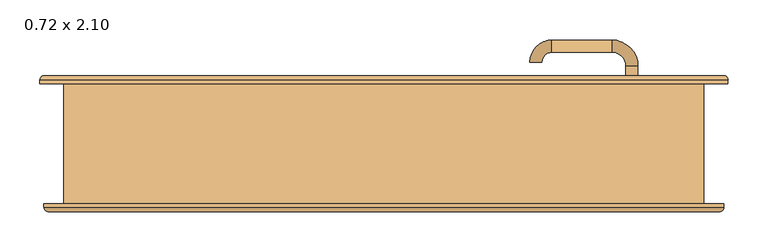
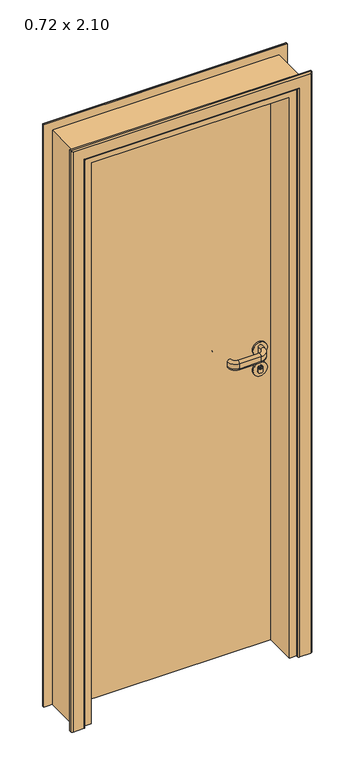
"""IFC4 building model written with IfcOpenShell, lengths in millimetres: door geometry, CC_PORTA ABRIR_1 FOLHA LISA : 0.72 x 2.10."""

from ifc_helpers import new_model, si_unit, point, frame, frame_2d, origin, origin_with_axes, place, context, project, spatial, polyline, circle_curve, ellipse_curve, trimmed, segment, composite_curve, outline, extrude, faceted_brep, source, transform, mapped, element, save
from ifc_brep_helpers import plane_surface, cylinder_surface, revolved_surface, advanced_brep


def door_0_72_x_2_10_9be13891(model_context):
    return source(origin(), model_context, "Body", "SolidModel", [
        advanced_brep(
        [(302.5, 40.0, 1091.5062746), (302.5, 40.0, 1108.3826844), (317.5, 40.0, 1108.3826844), (317.5, 40.0, 1091.5062746), (317.5, 18.0, 1108.3826844), (317.5, 18.0, 1091.5062746), (302.5, 18.0, 1091.5062746), (302.5, 18.0, 1108.3826844), (285.0, -14.5, 1108.3826844), (210.0, -14.5, 1108.3826844), (210.0, -14.5, 1091.5062746), (285.0, -14.5, 1091.5062746), (285.0, 0.5, 1091.5062746), (210.0, 0.5, 1091.5062746), (210.0, 0.5, 1108.3826844), (285.0, 0.5, 1108.3826844), (197.5, 13.0, 1091.5062746), (182.5, 13.0, 1091.5062746), (182.5, 13.0, 1108.3826844), (197.5, 13.0, 1108.3826844)],
        [
            (0, 1),
            (1, 2, circle_curve(frame((310.0, 40.0, 1108.3826844), z_axis=(0.0, 1.0, 0.0), x_axis=(0.0, 0.0, 1.0)), 7.5)),
            (2, 3),
            (3, 0, circle_curve(frame((310.0, 40.0, 1091.5062746), z_axis=(0.0, 1.0, 0.0), x_axis=(0.0, 0.0, 1.0)), 7.5)),
            (2, 4),
            (4, 5),
            (5, 3),
            (0, 6),
            (6, 7),
            (7, 1),
            (8, 9),
            (9, 10),
            (10, 11),
            (11, 8),
            (12, 13),
            (13, 14),
            (14, 15),
            (15, 12),
            (5, 6, circle_curve(frame((310.0, 18.0, 1091.5062746), z_axis=(0.0, 1.0, 0.0), x_axis=(0.0, 0.0, 1.0)), 7.5)),
            (7, 4, circle_curve(frame((310.0, 18.0, 1108.3826844), z_axis=(0.0, 1.0, 0.0), x_axis=(0.0, 0.0, 1.0)), 7.5)),
            (10, 13, circle_curve(frame((210.0, -7.0, 1091.5062746), z_axis=(1.0, 0.0, 0.0), x_axis=(0.0, 0.0, 1.0)), 7.5)),
            (12, 11, circle_curve(frame((285.0, -7.0, 1091.5062746), z_axis=(-1.0, 0.0, 0.0), x_axis=(0.0, 0.0, 1.0)), 7.5)),
            (14, 9, circle_curve(frame((210.0, -7.0, 1108.3826844), z_axis=(1.0, 0.0, 0.0), x_axis=(0.0, 0.0, 1.0)), 7.5)),
            (8, 15, circle_curve(frame((285.0, -7.0, 1108.3826844), z_axis=(-1.0, 0.0, 0.0), x_axis=(0.0, 0.0, 1.0)), 7.5)),
            (12, 6, circle_curve(frame((285.0, 18.0, 1091.5062746), z_axis=(0.0, 0.0, 1.0), x_axis=(1.0, 0.0, 0.0)), 17.5)),
            (5, 11, circle_curve(frame((285.0, 18.0, 1091.5062746), z_axis=(0.0, 0.0, -1.0), x_axis=(1.0, 0.0, 0.0)), 32.5)),
            (4, 8, circle_curve(frame((285.0, 18.0, 1108.3826844), z_axis=(0.0, 0.0, -1.0), x_axis=(1.0, 0.0, 0.0)), 32.5)),
            (7, 15, circle_curve(frame((285.0, 18.0, 1108.3826844), z_axis=(0.0, 0.0, -1.0), x_axis=(1.0, 0.0, 0.0)), 17.5)),
            (16, 17, circle_curve(frame((190.0, 13.0, 1091.5062746), z_axis=(0.0, 1.0, 0.0), x_axis=(0.0, 0.0, 1.0)), 7.5)),
            (17, 18),
            (18, 19, circle_curve(frame((190.0, 13.0, 1108.3826844), z_axis=(0.0, 1.0, 0.0), x_axis=(0.0, 0.0, 1.0)), 7.5)),
            (19, 16),
            (16, 13, circle_curve(frame((210.0, 13.0, 1091.5062746), z_axis=(0.0, 0.0, 1.0), x_axis=(0.0, -1.0, 0.0)), 12.5)),
            (10, 17, circle_curve(frame((210.0, 13.0, 1091.5062746), z_axis=(0.0, 0.0, -1.0), x_axis=(0.0, -1.0, 0.0)), 27.5)),
            (9, 18, circle_curve(frame((210.0, 13.0, 1108.3826844), z_axis=(0.0, 0.0, -1.0), x_axis=(0.0, -1.0, 0.0)), 27.5)),
            (14, 19, circle_curve(frame((210.0, 13.0, 1108.3826844), z_axis=(0.0, 0.0, -1.0), x_axis=(0.0, -1.0, 0.0)), 12.5)),
        ],
        [
            plane_surface(frame((310.0, 40.0, 1099.9444795), z_axis=(0.0, 1.0, 0.0), x_axis=(0.0, 0.0, 1.0))),
            plane_surface(frame((317.5, 40.0, 1091.5062746), z_axis=(1.0, 0.0, 0.0), x_axis=(0.0, -1.0, 0.0))),
            plane_surface(frame((302.5, 40.0, 1108.3826844), z_axis=(-1.0, 0.0, 0.0), x_axis=(0.0, -1.0, 0.0))),
            plane_surface(frame((285.0, -14.5, 1091.5062746), z_axis=(0.0, -1.0, 0.0), x_axis=(-1.0, 0.0, 0.0))),
            plane_surface(frame((285.0, 0.5, 1108.3826844), z_axis=(0.0, 1.0, 0.0), x_axis=(-1.0, 0.0, 0.0))),
            cylinder_surface(frame((310.0, 40.0, 1091.5062746), z_axis=(0.0, 1.0, 0.0), x_axis=(0.0, 0.0, 1.0)), 7.5),
            cylinder_surface(frame((310.0, 40.0, 1108.3826844), z_axis=(0.0, 1.0, 0.0), x_axis=(0.0, 0.0, 1.0)), 7.5),
            cylinder_surface(frame((285.0, -7.0, 1091.5062746), z_axis=(1.0, 0.0, 0.0), x_axis=(0.0, 0.0, 1.0)), 7.5),
            cylinder_surface(frame((285.0, -7.0, 1108.3826844), z_axis=(1.0, 0.0, 0.0), x_axis=(0.0, 0.0, 1.0)), 7.5),
            revolved_surface(trimmed(ellipse_curve(frame((310.0, 18.0, 1091.5062746), z_axis=(0.0, -1.0, 0.0), x_axis=(0.0, 0.0, 1.0)), 7.5, 7.5), [point((302.5, 18.0, 1091.5062746))], [point((317.5, 18.0, 1091.5062746))], True, "CARTESIAN"), (285.0, 18.0, 1099.9444795), (0.0, 0.0, 1.0)),
            cylinder_surface(frame((285.0, 18.0, 1099.9444795), z_axis=(0.0, 0.0, 1.0), x_axis=(1.0, 0.0, 0.0)), 32.5),
            revolved_surface(trimmed(ellipse_curve(frame((310.0, 18.0, 1108.3826844), z_axis=(0.0, -1.0, 0.0), x_axis=(0.0, 0.0, 1.0)), 7.5, 7.5), [point((317.5, 18.0, 1108.3826844))], [point((302.5, 18.0, 1108.3826844))], True, "CARTESIAN"), (285.0, 18.0, 1099.9444795), (0.0, 0.0, 1.0)),
            revolved_surface(polyline([(302.5, 18.0, 1108.3826844), (302.5, 18.0, 1091.5062746)]), (285.0, 18.0, 1099.9444795), (0.0, 0.0, 1.0)),
            plane_surface(frame((190.0, 13.0, 1099.9444795), z_axis=(0.0, 1.0, 0.0), x_axis=(0.0, 0.0, 1.0))),
            revolved_surface(trimmed(ellipse_curve(frame((210.0, -7.0, 1091.5062746), z_axis=(-1.0, 0.0, 0.0), x_axis=(0.0, 0.0, 1.0)), 7.5, 7.5), [point((210.0, 0.5, 1091.5062746))], [point((210.0, -14.5, 1091.5062746))], True, "CARTESIAN"), (210.0, 13.0, 1099.9444795), (0.0, 0.0, 1.0)),
            cylinder_surface(frame((210.0, 13.0, 1099.9444795), z_axis=(0.0, 0.0, 1.0), x_axis=(0.0, -1.0, 0.0)), 27.5),
            revolved_surface(trimmed(ellipse_curve(frame((210.0, -7.0, 1108.3826844), z_axis=(-1.0, 0.0, 0.0), x_axis=(0.0, 0.0, 1.0)), 7.5, 7.5), [point((210.0, -14.5, 1108.3826844))], [point((210.0, 0.5, 1108.3826844))], True, "CARTESIAN"), (210.0, 13.0, 1099.9444795), (0.0, 0.0, 1.0)),
            revolved_surface(polyline([(210.0, 0.5, 1108.3826844), (210.0, 0.5, 1091.5062746)]), (210.0, 13.0, 1099.9444795), (0.0, 0.0, 1.0)),
        ],
        [
            (0, [[1, 2, 3, 4]]),
            (1, [[5, 6, 7, -3]]),
            (2, [[8, 9, 10, -1]]),
            (3, [[11, 12, 13, 14]]),
            (4, [[15, 16, 17, 18]]),
            (5, [[-7, 19, -8, -4]]),
            (6, [[-10, 20, -5, -2]]),
            (7, [[-13, 21, -15, 22]]),
            (8, [[-17, 23, -11, 24]]),
            (9, [[-22, 25, -19, 26]]),
            (10, [[-14, -26, -6, 27]]),
            (11, [[-24, -27, -20, 28]]),
            (12, [[-18, -28, -9, -25]]),
            (13, [[29, 30, 31, 32]]),
            (14, [[-29, 33, -21, 34]]),
            (15, [[-30, -34, -12, 35]]),
            (16, [[-31, -35, -23, 36]]),
            (17, [[-32, -36, -16, -33]]),
        ],
    ),
        extrude(outline(polyline([(311.0, 40.0), (311.0, 30.9), (309.0, 30.9), (309.0, 40.0), (311.0, 40.0)])), frame((0.0, 0.0, 1027.9555433), z_axis=(0.0, 0.0, 1.0), x_axis=(1.0, 0.0, 0.0)), (0.0, 0.0, 1.0), 7.8071257),
        extrude(outline(composite_curve([segment(trimmed(circle_curve(frame_2d((1031.5611613, 310.0)), 5.0), [point((1036.5611613, 310.0))], [point((1026.5611613, 310.0))], False, "CARTESIAN"), True, "CONTINUOUS"), segment(trimmed(circle_curve(frame_2d((1031.5611613, 310.0)), 5.0), [point((1026.5611613, 310.0))], [point((1036.5611613, 310.0))], False, "CARTESIAN"), True, "CONTINUOUS")], self_intersect=False), holes=[polyline([(1035.7626689, 311.0), (1027.9555433, 311.0), (1027.9555433, 309.0), (1035.7626689, 309.0), (1035.7626689, 311.0)])]), frame((0.0, 30.0, 0.0), z_axis=(0.0, 1.0, 0.0), x_axis=(0.0, 0.0, 1.0)), (0.0, 0.0, 1.0), 10.0),
        extrude(outline(composite_curve([segment(polyline([(1033.4817325, 302.5), (1016.4817325, 302.5)]), True, "CONTINUOUS"), segment(trimmed(circle_curve(frame_2d((1016.4817325, 306.5)), 4.0), [point((1016.4817325, 302.5))], [point((1012.4817325, 306.5))], False, "CARTESIAN"), True, "CONTINUOUS"), segment(polyline([(1012.4817325, 306.5), (1012.4817325, 313.5)]), True, "CONTINUOUS"), segment(trimmed(circle_curve(frame_2d((1016.4817325, 313.5)), 4.0), [point((1012.4817325, 313.5))], [point((1016.4817325, 317.5))], False, "CARTESIAN"), True, "CONTINUOUS"), segment(polyline([(1016.4817325, 317.5), (1033.4817325, 317.5)]), True, "CONTINUOUS"), segment(trimmed(circle_curve(frame_2d((1033.4817325, 313.5)), 4.0), [point((1033.4817325, 317.5))], [point((1037.4817325, 313.5))], False, "CARTESIAN"), True, "CONTINUOUS"), segment(polyline([(1037.4817325, 313.5), (1037.4817325, 306.5)]), True, "CONTINUOUS"), segment(trimmed(circle_curve(frame_2d((1033.4817325, 306.5)), 4.0), [point((1037.4817325, 306.5))], [point((1033.4817325, 302.5))], False, "CARTESIAN"), True, "CONTINUOUS")], self_intersect=False)), frame((0.0, 31.0, 0.0), z_axis=(0.0, 1.0, 0.0), x_axis=(0.0, 0.0, 1.0)), (0.0, 0.0, 1.0), 9.0),
        extrude(outline(composite_curve([segment(trimmed(circle_curve(frame_2d((1099.9444795, 310.0)), 25.0), [point((1124.9444795, 310.0))], [point((1074.9444795, 310.0))], False, "CARTESIAN"), True, "CONTINUOUS"), segment(trimmed(circle_curve(frame_2d((1099.9444795, 310.0)), 25.0), [point((1074.9444795, 310.0))], [point((1124.9444795, 310.0))], False, "CARTESIAN"), True, "CONTINUOUS")], self_intersect=False)), frame((0.0, 34.0, 0.0), z_axis=(0.0, 1.0, 0.0), x_axis=(0.0, 0.0, 1.0)), (0.0, 0.0, 1.0), 6.0),
        extrude(outline(composite_curve([segment(trimmed(circle_curve(frame_2d((1024.9444795, 310.0)), 25.0), [point((1049.9444795, 310.0))], [point((999.9444795, 310.0))], False, "CARTESIAN"), True, "CONTINUOUS"), segment(trimmed(circle_curve(frame_2d((1024.9444795, 310.0)), 25.0), [point((999.9444795, 310.0))], [point((1049.9444795, 310.0))], False, "CARTESIAN"), True, "CONTINUOUS")], self_intersect=False), holes=[composite_curve([segment(trimmed(circle_curve(frame_2d((1033.4817325, 313.5)), 4.0), [point((1037.4817325, 313.5))], [point((1033.4817325, 317.5))], True, "CARTESIAN"), True, "CONTINUOUS"), segment(polyline([(1033.4817325, 317.5), (1016.4817325, 317.5)]), True, "CONTINUOUS"), segment(trimmed(circle_curve(frame_2d((1016.4817325, 313.5)), 4.0), [point((1016.4817325, 317.5))], [point((1012.4817325, 313.5))], True, "CARTESIAN"), True, "CONTINUOUS"), segment(polyline([(1012.4817325, 313.5), (1012.4817325, 306.5)]), True, "CONTINUOUS"), segment(trimmed(circle_curve(frame_2d((1016.4817325, 306.5)), 4.0), [point((1012.4817325, 306.5))], [point((1016.4817325, 302.5))], True, "CARTESIAN"), True, "CONTINUOUS"), segment(polyline([(1016.4817325, 302.5), (1033.4817325, 302.5)]), True, "CONTINUOUS"), segment(trimmed(circle_curve(frame_2d((1033.4817325, 306.5)), 4.0), [point((1033.4817325, 302.5))], [point((1037.4817325, 306.5))], True, "CARTESIAN"), True, "CONTINUOUS"), segment(polyline([(1037.4817325, 306.5), (1037.4817325, 313.5)]), True, "CONTINUOUS")], self_intersect=False)]), frame((0.0, 34.0, 0.0), z_axis=(0.0, 1.0, 0.0), x_axis=(0.0, 0.0, 1.0)), (0.0, 0.0, 1.0), 6.0),
        extrude(outline(polyline([(311.0, 84.1), (311.0, 75.0), (309.0, 75.0), (309.0, 84.1), (311.0, 84.1)])), frame((0.0, 0.0, 1027.9555433), z_axis=(0.0, 0.0, 1.0), x_axis=(1.0, 0.0, 0.0)), (0.0, 0.0, 1.0), 7.8071257),
        advanced_brep(
        [(310.0, 85.0, 1036.5611613), (310.0, 85.0, 1026.5611613), (311.0, 85.0, 1035.7626689), (309.0, 85.0, 1035.7626689), (309.0, 85.0, 1027.9555433), (311.0, 85.0, 1027.9555433), (310.0, 75.0, 1049.9444795), (310.0, 75.0, 999.9444795), (310.0, 84.0, 1026.5611613), (310.0, 84.0, 1036.5611613), (311.0, 84.0, 1027.9555433), (311.0, 84.0, 1035.7626689), (309.0, 84.0, 1027.9555433), (309.0, 84.0, 1035.7626689), (302.5, 84.0, 1033.4817325), (306.5, 84.0, 1037.4817325), (313.5, 84.0, 1037.4817325), (317.5, 84.0, 1033.4817325), (317.5, 84.0, 1016.4817325), (313.5, 84.0, 1012.4817325), (306.5, 84.0, 1012.4817325), (302.5, 84.0, 1016.4817325), (302.5, 81.0, 1016.4817325), (302.5, 81.0, 1033.4817325), (306.5, 81.0, 1012.4817325), (313.5, 81.0, 1012.4817325), (317.5, 81.0, 1016.4817325), (317.5, 81.0, 1033.4817325), (313.5, 81.0, 1037.4817325), (306.5, 81.0, 1037.4817325), (310.0, 81.0, 1049.9444795), (310.0, 81.0, 999.9444795)],
        [
            (0, 1, circle_curve(frame((310.0, 85.0, 1031.5611613), z_axis=(0.0, 1.0, 0.0), x_axis=(0.0, 0.0, -1.0)), 5.0)),
            (1, 0, circle_curve(frame((310.0, 85.0, 1031.5611613), z_axis=(0.0, 1.0, 0.0), x_axis=(0.0, 0.0, -1.0)), 5.0)),
            (2, 3),
            (3, 4),
            (4, 5),
            (5, 2),
            (6, 7, circle_curve(frame((310.0, 75.0, 1024.9444795), z_axis=(0.0, -1.0, 0.0), x_axis=(0.0, 0.0, -1.0)), 25.0)),
            (7, 6, circle_curve(frame((310.0, 75.0, 1024.9444795), z_axis=(0.0, -1.0, 0.0), x_axis=(0.0, 0.0, -1.0)), 25.0)),
            (1, 8),
            (8, 9, circle_curve(frame((310.0, 84.0, 1031.5611613), z_axis=(0.0, 1.0, 0.0), x_axis=(0.0, 0.0, -1.0)), 5.0)),
            (9, 0),
            (9, 8, circle_curve(frame((310.0, 84.0, 1031.5611613), z_axis=(0.0, 1.0, 0.0), x_axis=(0.0, 0.0, -1.0)), 5.0)),
            (5, 10),
            (10, 11),
            (11, 2),
            (4, 12),
            (12, 10),
            (3, 13),
            (13, 12),
            (11, 13),
            (14, 15, circle_curve(frame((306.5, 84.0, 1033.4817325), z_axis=(0.0, 1.0, 0.0), x_axis=(0.0, 0.0, -1.0)), 4.0)),
            (15, 16),
            (16, 17, circle_curve(frame((313.5, 84.0, 1033.4817325), z_axis=(0.0, 1.0, 0.0), x_axis=(0.0, 0.0, -1.0)), 4.0)),
            (17, 18),
            (18, 19, circle_curve(frame((313.5, 84.0, 1016.4817325), z_axis=(0.0, 1.0, 0.0), x_axis=(0.0, 0.0, -1.0)), 4.0)),
            (19, 20),
            (20, 21, circle_curve(frame((306.5, 84.0, 1016.4817325), z_axis=(0.0, 1.0, 0.0), x_axis=(0.0, 0.0, -1.0)), 4.0)),
            (21, 14),
            (21, 22),
            (22, 23),
            (23, 14),
            (20, 24),
            (24, 22, circle_curve(frame((306.5, 81.0, 1016.4817325), z_axis=(0.0, 1.0, 0.0), x_axis=(0.0, 0.0, -1.0)), 4.0)),
            (19, 25),
            (25, 24),
            (18, 26),
            (26, 25, circle_curve(frame((313.5, 81.0, 1016.4817325), z_axis=(0.0, 1.0, 0.0), x_axis=(0.0, 0.0, -1.0)), 4.0)),
            (17, 27),
            (27, 26),
            (16, 28),
            (28, 27, circle_curve(frame((313.5, 81.0, 1033.4817325), z_axis=(0.0, 1.0, 0.0), x_axis=(0.0, 0.0, -1.0)), 4.0)),
            (15, 29),
            (29, 28),
            (23, 29, circle_curve(frame((306.5, 81.0, 1033.4817325), z_axis=(0.0, 1.0, 0.0), x_axis=(0.0, 0.0, -1.0)), 4.0)),
            (30, 31, circle_curve(frame((310.0, 81.0, 1024.9444795), z_axis=(0.0, 1.0, 0.0), x_axis=(0.0, 0.0, -1.0)), 25.0)),
            (31, 30, circle_curve(frame((310.0, 81.0, 1024.9444795), z_axis=(0.0, 1.0, 0.0), x_axis=(0.0, 0.0, -1.0)), 25.0)),
            (31, 7),
            (6, 30),
        ],
        [
            plane_surface(frame((310.0, 85.0, 1026.5611613), z_axis=(0.0, 1.0, 0.0), x_axis=(1.0, 0.0, 0.0))),
            plane_surface(frame((310.0, 75.0, 1026.5611613), z_axis=(0.0, -1.0, 0.0), x_axis=(-1.0, 0.0, 0.0))),
            cylinder_surface(frame((310.0, 75.0, 1031.5611613), z_axis=(0.0, 1.0, 0.0), x_axis=(0.0, 0.0, -1.0)), 5.0),
            plane_surface(frame((311.0, 85.0, 1035.7626689), z_axis=(-1.0, 0.0, 0.0), x_axis=(0.0, -1.0, 0.0))),
            plane_surface(frame((311.0, 85.0, 1027.9555433), z_axis=(0.0, 0.0, 1.0), x_axis=(0.0, -1.0, 0.0))),
            plane_surface(frame((309.0, 85.0, 1027.9555433), z_axis=(1.0, 0.0, 0.0), x_axis=(0.0, -1.0, 0.0))),
            plane_surface(frame((309.0, 85.0, 1035.7626689), z_axis=(0.0, 0.0, -1.0), x_axis=(0.0, -1.0, 0.0))),
            plane_surface(frame((302.5, 84.0, 1016.4817325), z_axis=(0.0, 1.0, 0.0), x_axis=(0.0, 0.0, -1.0))),
            plane_surface(frame((302.5, 84.0, 1033.4817325), z_axis=(-1.0, 0.0, 0.0), x_axis=(0.0, -1.0, 0.0))),
            cylinder_surface(frame((306.5, 75.0, 1016.4817325), z_axis=(0.0, 1.0, 0.0), x_axis=(0.0, 0.0, -1.0)), 4.0),
            plane_surface(frame((306.5, 84.0, 1012.4817325), z_axis=(0.0, 0.0, -1.0), x_axis=(0.0, -1.0, 0.0))),
            cylinder_surface(frame((313.5, 75.0, 1016.4817325), z_axis=(0.0, 1.0, 0.0), x_axis=(0.0, 0.0, -1.0)), 4.0),
            plane_surface(frame((317.5, 84.0, 1016.4817325), z_axis=(1.0, 0.0, 0.0), x_axis=(0.0, -1.0, 0.0))),
            cylinder_surface(frame((313.5, 75.0, 1033.4817325), z_axis=(0.0, 1.0, 0.0), x_axis=(0.0, 0.0, -1.0)), 4.0),
            plane_surface(frame((313.5, 84.0, 1037.4817325), z_axis=(0.0, 0.0, 1.0), x_axis=(0.0, -1.0, 0.0))),
            cylinder_surface(frame((306.5, 75.0, 1033.4817325), z_axis=(0.0, 1.0, 0.0), x_axis=(0.0, 0.0, -1.0)), 4.0),
            plane_surface(frame((310.0, 81.0, 1074.9444795), z_axis=(0.0, 1.0, 0.0), x_axis=(1.0, 0.0, 0.0))),
            cylinder_surface(frame((310.0, 75.0, 1024.9444795), z_axis=(0.0, 1.0, 0.0), x_axis=(0.0, 0.0, -1.0)), 25.0),
        ],
        [
            (0, [[1, 2], [3, 4, 5, 6]]),
            (1, [[7, 8]]),
            (2, [[9, 10, 11, -2]]),
            (2, [[-11, 12, -9, -1]]),
            (3, [[13, 14, 15, -6]]),
            (4, [[16, 17, -13, -5]]),
            (5, [[18, 19, -16, -4]]),
            (6, [[-15, 20, -18, -3]]),
            (7, [[-17, -19, -20, -14]]),
            (7, [[21, 22, 23, 24, 25, 26, 27, 28], [-12, -10]]),
            (8, [[29, 30, 31, -28]]),
            (9, [[32, 33, -29, -27]]),
            (10, [[34, 35, -32, -26]]),
            (11, [[36, 37, -34, -25]]),
            (12, [[38, 39, -36, -24]]),
            (13, [[40, 41, -38, -23]]),
            (14, [[42, 43, -40, -22]]),
            (15, [[-31, 44, -42, -21]]),
            (16, [[45, 46], [-33, -35, -37, -39, -41, -43, -44, -30]]),
            (17, [[47, -7, 48, -46]]),
            (17, [[-48, -8, -47, -45]]),
        ],
    ),
        advanced_brep(
        [(310.0, 75.0, 1124.9444795), (310.0, 75.0, 1074.9444795), (310.0, 81.0, 1124.9444795), (310.0, 81.0, 1074.9444795)],
        [
            (0, 1, circle_curve(frame((310.0, 75.0, 1099.9444795), z_axis=(0.0, -1.0, 0.0), x_axis=(0.0, 0.0, -1.0)), 25.0)),
            (1, 0, circle_curve(frame((310.0, 75.0, 1099.9444795), z_axis=(0.0, -1.0, 0.0), x_axis=(0.0, 0.0, -1.0)), 25.0)),
            (2, 3, circle_curve(frame((310.0, 81.0, 1099.9444795), z_axis=(0.0, 1.0, 0.0), x_axis=(0.0, 0.0, -1.0)), 25.0)),
            (3, 2, circle_curve(frame((310.0, 81.0, 1099.9444795), z_axis=(0.0, 1.0, 0.0), x_axis=(0.0, 0.0, -1.0)), 25.0)),
            (3, 1),
            (0, 2),
        ],
        [
            plane_surface(frame((310.0, 75.0, 1026.5611613), z_axis=(0.0, -1.0, 0.0), x_axis=(-1.0, 0.0, 0.0))),
            plane_surface(frame((310.0, 81.0, 1074.9444795), z_axis=(0.0, 1.0, 0.0), x_axis=(1.0, 0.0, 0.0))),
            cylinder_surface(frame((310.0, 75.0, 1099.9444795), z_axis=(0.0, 1.0, 0.0), x_axis=(0.0, 0.0, -1.0)), 25.0),
        ],
        [
            (0, [[1, 2]]),
            (1, [[3, 4]]),
            (2, [[5, -1, 6, -4]]),
            (2, [[-6, -2, -5, -3]]),
        ],
    ),
        advanced_brep(
        [(302.5, 75.0, 1108.4382049), (302.5, 75.0, 1091.5617951), (317.5, 75.0, 1091.5617951), (317.5, 75.0, 1108.4382049), (317.5, 97.0, 1091.5617951), (317.5, 97.0, 1108.4382049), (302.5, 97.0, 1108.4382049), (302.5, 97.0, 1091.5617951), (285.0, 129.5, 1091.5617951), (210.0, 129.5, 1091.5617951), (210.0, 129.5, 1108.4382049), (285.0, 129.5, 1108.4382049), (285.0, 114.5, 1108.4382049), (210.0, 114.5, 1108.4382049), (210.0, 114.5, 1091.5617951), (285.0, 114.5, 1091.5617951), (197.5, 102.0, 1108.4382049), (182.5, 102.0, 1108.4382049), (182.5, 102.0, 1091.5617951), (197.5, 102.0, 1091.5617951)],
        [
            (0, 1),
            (1, 2, circle_curve(frame((310.0, 75.0, 1091.5617951), z_axis=(0.0, -1.0, 0.0), x_axis=(-1.0, 0.0, 0.0)), 7.5)),
            (2, 3),
            (3, 0, circle_curve(frame((310.0, 75.0, 1108.4382049), z_axis=(0.0, -1.0, 0.0), x_axis=(-1.0, 0.0, 0.0)), 7.5)),
            (2, 4),
            (4, 5),
            (5, 3),
            (0, 6),
            (6, 7),
            (7, 1),
            (8, 9),
            (9, 10),
            (10, 11),
            (11, 8),
            (12, 13),
            (13, 14),
            (14, 15),
            (15, 12),
            (5, 6, circle_curve(frame((310.0, 97.0, 1108.4382049), z_axis=(0.0, -1.0, 0.0), x_axis=(-1.0, 0.0, 0.0)), 7.5)),
            (7, 4, circle_curve(frame((310.0, 97.0, 1091.5617951), z_axis=(0.0, -1.0, 0.0), x_axis=(-1.0, 0.0, 0.0)), 7.5)),
            (10, 13, circle_curve(frame((210.0, 122.0, 1108.4382049), z_axis=(1.0, 0.0, 0.0), x_axis=(0.0, -1.0, 0.0)), 7.5)),
            (12, 11, circle_curve(frame((285.0, 122.0, 1108.4382049), z_axis=(-1.0, 0.0, 0.0), x_axis=(0.0, -1.0, 0.0)), 7.5)),
            (14, 9, circle_curve(frame((210.0, 122.0, 1091.5617951), z_axis=(1.0, 0.0, 0.0), x_axis=(0.0, -1.0, 0.0)), 7.5)),
            (8, 15, circle_curve(frame((285.0, 122.0, 1091.5617951), z_axis=(-1.0, 0.0, 0.0), x_axis=(0.0, -1.0, 0.0)), 7.5)),
            (12, 6, circle_curve(frame((285.0, 97.0, 1108.4382049), z_axis=(0.0, 0.0, -1.0), x_axis=(1.0, 0.0, 0.0)), 17.5)),
            (5, 11, circle_curve(frame((285.0, 97.0, 1108.4382049), z_axis=(0.0, 0.0, 1.0), x_axis=(1.0, 0.0, 0.0)), 32.5)),
            (4, 8, circle_curve(frame((285.0, 97.0, 1091.5617951), z_axis=(0.0, 0.0, 1.0), x_axis=(1.0, 0.0, 0.0)), 32.5)),
            (7, 15, circle_curve(frame((285.0, 97.0, 1091.5617951), z_axis=(0.0, 0.0, 1.0), x_axis=(1.0, 0.0, 0.0)), 17.5)),
            (16, 17, circle_curve(frame((190.0, 102.0, 1108.4382049), z_axis=(0.0, -1.0, 0.0), x_axis=(1.0, 0.0, 0.0)), 7.5)),
            (17, 18),
            (18, 19, circle_curve(frame((190.0, 102.0, 1091.5617951), z_axis=(0.0, -1.0, 0.0), x_axis=(1.0, 0.0, 0.0)), 7.5)),
            (19, 16),
            (16, 13, circle_curve(frame((210.0, 102.0, 1108.4382049), z_axis=(0.0, 0.0, -1.0), x_axis=(0.0, 1.0, 0.0)), 12.5)),
            (10, 17, circle_curve(frame((210.0, 102.0, 1108.4382049), z_axis=(0.0, 0.0, 1.0), x_axis=(0.0, 1.0, 0.0)), 27.5)),
            (9, 18, circle_curve(frame((210.0, 102.0, 1091.5617951), z_axis=(0.0, 0.0, 1.0), x_axis=(0.0, 1.0, 0.0)), 27.5)),
            (14, 19, circle_curve(frame((210.0, 102.0, 1091.5617951), z_axis=(0.0, 0.0, 1.0), x_axis=(0.0, 1.0, 0.0)), 12.5)),
        ],
        [
            plane_surface(frame((310.0, 75.0, 1100.0), z_axis=(0.0, -1.0, 0.0), x_axis=(0.0, 0.0, -1.0))),
            plane_surface(frame((317.5, 75.0, 1108.4382049), z_axis=(1.0, 0.0, 0.0), x_axis=(0.0, 1.0, 0.0))),
            plane_surface(frame((302.5, 75.0, 1091.5617951), z_axis=(-1.0, 0.0, 0.0), x_axis=(0.0, 1.0, 0.0))),
            plane_surface(frame((285.0, 129.5, 1108.4382049), z_axis=(0.0, 1.0, 0.0), x_axis=(-1.0, 0.0, 0.0))),
            plane_surface(frame((285.0, 114.5, 1091.5617951), z_axis=(0.0, -1.0, 0.0), x_axis=(-1.0, 0.0, 0.0))),
            cylinder_surface(frame((310.0, 75.0, 1108.4382049), z_axis=(0.0, -1.0, 0.0), x_axis=(-1.0, 0.0, 0.0)), 7.5),
            cylinder_surface(frame((310.0, 75.0, 1091.5617951), z_axis=(0.0, -1.0, 0.0), x_axis=(-1.0, 0.0, 0.0)), 7.5),
            cylinder_surface(frame((285.0, 122.0, 1108.4382049), z_axis=(1.0, 0.0, 0.0), x_axis=(0.0, -1.0, 0.0)), 7.5),
            cylinder_surface(frame((285.0, 122.0, 1091.5617951), z_axis=(1.0, 0.0, 0.0), x_axis=(0.0, -1.0, 0.0)), 7.5),
            revolved_surface(trimmed(ellipse_curve(frame((310.0, 97.0, 1108.4382049), z_axis=(0.0, 1.0, 0.0), x_axis=(-1.0, 0.0, 0.0)), 7.5, 7.5), [point((302.5, 97.0, 1108.4382049))], [point((317.5, 97.0, 1108.4382049))], True, "CARTESIAN"), (285.0, 97.0, 1100.0), (0.0, 0.0, -1.0)),
            cylinder_surface(frame((285.0, 97.0, 1100.0), z_axis=(0.0, 0.0, -1.0), x_axis=(1.0, 0.0, 0.0)), 32.5),
            revolved_surface(trimmed(ellipse_curve(frame((310.0, 97.0, 1091.5617951), z_axis=(0.0, 1.0, 0.0), x_axis=(-1.0, 0.0, 0.0)), 7.5, 7.5), [point((317.5, 97.0, 1091.5617951))], [point((302.5, 97.0, 1091.5617951))], True, "CARTESIAN"), (285.0, 97.0, 1100.0), (0.0, 0.0, -1.0)),
            revolved_surface(polyline([(302.5, 97.0, 1091.5617951), (302.5, 97.0, 1108.4382049)]), (285.0, 97.0, 1100.0), (0.0, 0.0, -1.0)),
            plane_surface(frame((190.0, 102.0, 1100.0), z_axis=(0.0, -1.0, 0.0), x_axis=(0.0, 0.0, -1.0))),
            revolved_surface(trimmed(ellipse_curve(frame((210.0, 122.0, 1108.4382049), z_axis=(-1.0, 0.0, 0.0), x_axis=(0.0, -1.0, 0.0)), 7.5, 7.5), [point((210.0, 114.5, 1108.4382049))], [point((210.0, 129.5, 1108.4382049))], True, "CARTESIAN"), (210.0, 102.0, 1100.0), (0.0, 0.0, -1.0)),
            cylinder_surface(frame((210.0, 102.0, 1100.0), z_axis=(0.0, 0.0, -1.0), x_axis=(0.0, 1.0, 0.0)), 27.5),
            revolved_surface(trimmed(ellipse_curve(frame((210.0, 122.0, 1091.5617951), z_axis=(-1.0, 0.0, 0.0), x_axis=(0.0, -1.0, 0.0)), 7.5, 7.5), [point((210.0, 129.5, 1091.5617951))], [point((210.0, 114.5, 1091.5617951))], True, "CARTESIAN"), (210.0, 102.0, 1100.0), (0.0, 0.0, -1.0)),
            revolved_surface(polyline([(210.0, 114.5, 1091.5617951), (210.0, 114.5, 1108.4382049)]), (210.0, 102.0, 1100.0), (0.0, 0.0, -1.0)),
        ],
        [
            (0, [[1, 2, 3, 4]]),
            (1, [[5, 6, 7, -3]]),
            (2, [[8, 9, 10, -1]]),
            (3, [[11, 12, 13, 14]]),
            (4, [[15, 16, 17, 18]]),
            (5, [[-7, 19, -8, -4]]),
            (6, [[-10, 20, -5, -2]]),
            (7, [[-13, 21, -15, 22]]),
            (8, [[-17, 23, -11, 24]]),
            (9, [[-22, 25, -19, 26]]),
            (10, [[-14, -26, -6, 27]]),
            (11, [[-24, -27, -20, 28]]),
            (12, [[-18, -28, -9, -25]]),
            (13, [[29, 30, 31, 32]]),
            (14, [[-29, 33, -21, 34]]),
            (15, [[-30, -34, -12, 35]]),
            (16, [[-31, -35, -23, 36]]),
            (17, [[-32, -36, -16, -33]]),
        ],
    ),
        extrude(outline(polyline([(360.0, 75.0), (360.0, 40.0), (-360.0, 40.0), (-360.0, 75.0), (360.0, 75.0)])), origin_with_axes(), (0.0, 0.0, 1.0), 2100.0),
        advanced_brep(
        [(-380.5, -85.0, 0.0), (-419.500573, -85.0, 0.0), (-425.0, -79.500573, 0.0), (-425.0, -75.0, 0.0), (-375.0, -75.0, 0.0), (-375.0, -79.5, 0.0), (-375.0, -79.5, 2115.0), (-380.5, -85.0, 2120.5), (-375.0, -75.0, 2115.0), (-425.0, -75.0, 2165.0), (425.0, -75.0, 2165.0), (425.0, -75.0, 0.0), (375.0, -75.0, 0.0), (375.0, -75.0, 2115.0), (-425.0, -79.500573, 2165.0), (-419.500573, -85.0, 2159.500573), (380.5, -85.0, 2120.5), (380.5, -85.0, 0.0), (419.500573, -85.0, 0.0), (419.500573, -85.0, 2159.500573), (375.0, -79.5, 0.0), (375.0, -79.5, 2115.0), (425.0, -79.500573, 0.0), (425.0, -79.500573, 2165.0)],
        [
            (0, 1),
            (1, 2, circle_curve(frame((-419.500573, -79.500573, 0.0), z_axis=(0.0, 0.0, -1.0), x_axis=(0.0, -1.0, 0.0)), 5.499427)),
            (2, 3),
            (3, 4),
            (4, 5),
            (5, 0, circle_curve(frame((-380.5, -79.5, 0.0), z_axis=(0.0, 0.0, -1.0), x_axis=(0.0, -1.0, 0.0)), 5.5)),
            (5, 6),
            (6, 7, ellipse_curve(frame((-380.5, -79.5, 2120.5), z_axis=(-0.7071067811865475, 0.0, -0.7071067811865476), x_axis=(0.7071067811865476, 0.0, -0.7071067811865474)), 7.7781746, 5.5)),
            (7, 0),
            (4, 8),
            (8, 6),
            (3, 9),
            (9, 10),
            (10, 11),
            (11, 12),
            (12, 13),
            (13, 8),
            (2, 14),
            (14, 9),
            (1, 15),
            (15, 14, ellipse_curve(frame((-419.500573, -79.500573, 2159.500573), z_axis=(-0.7071067811865475, 0.0, -0.7071067811865476), x_axis=(0.7071067811865476, 0.0, -0.7071067811865474)), 7.7773642, 5.499427)),
            (7, 16),
            (16, 17),
            (17, 18),
            (18, 19),
            (19, 15),
            (12, 20),
            (20, 21),
            (21, 13),
            (17, 20, circle_curve(frame((380.5, -79.5, 0.0), z_axis=(0.0, 0.0, -1.0), x_axis=(0.0, -1.0, 0.0)), 5.5)),
            (11, 22),
            (22, 18, circle_curve(frame((419.500573, -79.500573, 0.0), z_axis=(0.0, 0.0, -1.0), x_axis=(0.0, -1.0, 0.0)), 5.499427)),
            (23, 22),
            (10, 23),
            (23, 19, ellipse_curve(frame((419.500573, -79.500573, 2159.500573), z_axis=(0.7071067811865475, 0.0, -0.7071067811865475), x_axis=(0.7071067811865474, 0.0, 0.7071067811865477)), 7.7773642, 5.499427)),
            (16, 21, ellipse_curve(frame((380.5, -79.5, 2120.5), z_axis=(0.7071067811865475, 0.0, -0.7071067811865475), x_axis=(0.7071067811865474, 0.0, 0.7071067811865477)), 7.7781746, 5.5)),
            (6, 21),
            (14, 23),
        ],
        [
            plane_surface(frame((-400.0, -75.0, 0.0), z_axis=(0.0, 0.0, -1.0), x_axis=(-1.0, 0.0, 0.0))),
            cylinder_surface(frame((-380.5, -79.5, 0.0), z_axis=(0.0, 0.0, -1.0), x_axis=(0.0, -1.0, 0.0)), 5.5),
            plane_surface(frame((-375.0, -79.5, 0.0), z_axis=(1.0, 0.0, 0.0), x_axis=(0.0, 0.0, 1.0))),
            plane_surface(frame((-375.0, -75.0, 0.0), z_axis=(0.0, 1.0, 0.0), x_axis=(0.0, 0.0, 1.0))),
            plane_surface(frame((-425.0, -75.0, 0.0), z_axis=(-1.0, 0.0, 0.0), x_axis=(0.0, 0.0, 1.0))),
            cylinder_surface(frame((-419.500573, -79.500573, 0.0), z_axis=(0.0, 0.0, -1.0), x_axis=(0.0, -1.0, 0.0)), 5.499427),
            plane_surface(frame((-419.500573, -85.0, 0.0), z_axis=(0.0, -1.0, 0.0), x_axis=(0.0, 0.0, 1.0))),
            plane_surface(frame((375.0, -79.5, 2115.0), z_axis=(-1.0, 0.0, 0.0), x_axis=(0.0, 0.0, -1.0))),
            plane_surface(frame((400.0, -75.0, 0.0), z_axis=(0.0, 0.0, -1.0), x_axis=(1.0, 0.0, 0.0))),
            plane_surface(frame((425.0, -75.0, 2165.0), z_axis=(1.0, 0.0, 0.0), x_axis=(0.0, 0.0, -1.0))),
            cylinder_surface(frame((419.500573, -79.500573, 2140.0), z_axis=(0.0, 0.0, 1.0), x_axis=(0.0, -1.0, 0.0)), 5.499427),
            cylinder_surface(frame((380.5, -79.5, 2140.0), z_axis=(0.0, 0.0, 1.0), x_axis=(0.0, -1.0, 0.0)), 5.5),
            cylinder_surface(frame((-400.0, -79.5, 2120.5), z_axis=(-1.0, 0.0, 0.0), x_axis=(0.0, -1.0, 0.0)), 5.5),
            plane_surface(frame((-375.0, -79.5, 2115.0), z_axis=(0.0, 0.0, -1.0), x_axis=(1.0, 0.0, 0.0))),
            plane_surface(frame((-425.0, -75.0, 2165.0), z_axis=(0.0, 0.0, 1.0), x_axis=(1.0, 0.0, 0.0))),
            cylinder_surface(frame((-400.0, -79.500573, 2159.500573), z_axis=(-1.0, 0.0, 0.0), x_axis=(0.0, -1.0, 0.0)), 5.499427),
        ],
        [
            (0, [[1, 2, 3, 4, 5, 6]]),
            (1, [[7, 8, 9, -6]]),
            (2, [[10, 11, -7, -5]]),
            (3, [[12, 13, 14, 15, 16, 17, -10, -4]]),
            (4, [[18, 19, -12, -3]]),
            (5, [[20, 21, -18, -2]]),
            (6, [[-9, 22, 23, 24, 25, 26, -20, -1]]),
            (7, [[-16, 27, 28, 29]]),
            (8, [[30, -27, -15, 31, 32, -24]]),
            (9, [[33, -31, -14, 34]]),
            (10, [[-25, -32, -33, 35]]),
            (11, [[-28, -30, -23, 36]]),
            (12, [[37, -36, -22, -8]]),
            (13, [[-17, -29, -37, -11]]),
            (14, [[38, -34, -13, -19]]),
            (15, [[-26, -35, -38, -21]]),
        ],
    ),
        advanced_brep(
        [(-380.0, 75.0, 0.0), (-430.0, 75.0, 0.0), (-430.0, 79.5, 0.0), (-424.5, 85.0, 0.0), (-385.5, 85.0, 0.0), (-380.0, 79.5, 0.0), (-380.0, 79.5, 2120.0), (-380.0, 75.0, 2120.0), (-385.5, 85.0, 2125.5), (-424.5, 85.0, 2164.5), (424.5, 85.0, 2164.5), (424.5, 85.0, 0.0), (385.5, 85.0, 0.0), (385.5, 85.0, 2125.5), (-430.0, 79.5, 2170.0), (-430.0, 75.0, 2170.0), (380.0, 75.0, 2120.0), (380.0, 75.0, 0.0), (430.0, 75.0, 0.0), (430.0, 75.0, 2170.0), (380.0, 79.5, 0.0), (380.0, 79.5, 2120.0), (430.0, 79.5, 0.0), (430.0, 79.5, 2170.0)],
        [
            (0, 1),
            (1, 2),
            (2, 3, circle_curve(frame((-424.5, 79.5, 0.0), z_axis=(0.0, 0.0, -1.0), x_axis=(0.0, -1.0, 0.0)), 5.5)),
            (3, 4),
            (4, 5, circle_curve(frame((-385.5, 79.5, 0.0), z_axis=(0.0, 0.0, -1.0), x_axis=(0.0, -1.0, 0.0)), 5.5)),
            (5, 0),
            (5, 6),
            (6, 7),
            (7, 0),
            (4, 8),
            (8, 6, ellipse_curve(frame((-385.5, 79.5, 2125.5), z_axis=(-0.7071067811865475, 0.0, -0.7071067811865476), x_axis=(0.7071067811865476, 0.0, -0.7071067811865474)), 7.7781746, 5.5)),
            (3, 9),
            (9, 10),
            (10, 11),
            (11, 12),
            (12, 13),
            (13, 8),
            (2, 14),
            (14, 9, ellipse_curve(frame((-424.5, 79.5, 2164.5), z_axis=(-0.7071067811865475, 0.0, -0.7071067811865476), x_axis=(0.7071067811865476, 0.0, -0.7071067811865474)), 7.7781746, 5.5)),
            (1, 15),
            (15, 14),
            (7, 16),
            (16, 17),
            (17, 18),
            (18, 19),
            (19, 15),
            (12, 20, circle_curve(frame((385.5, 79.5, 0.0), z_axis=(0.0, 0.0, 1.0), x_axis=(0.0, -1.0, 0.0)), 5.5)),
            (20, 21),
            (21, 13, ellipse_curve(frame((385.5, 79.5, 2125.5), z_axis=(0.7071067811865475, 0.0, -0.7071067811865475), x_axis=(0.7071067811865474, 0.0, 0.7071067811865477)), 7.7781746, 5.5)),
            (17, 20),
            (11, 22, circle_curve(frame((424.5, 79.5, 0.0), z_axis=(0.0, 0.0, -1.0), x_axis=(0.0, -1.0, 0.0)), 5.5)),
            (22, 18),
            (23, 22),
            (10, 23, ellipse_curve(frame((424.5, 79.5, 2164.5), z_axis=(0.7071067811865475, 0.0, -0.7071067811865475), x_axis=(0.7071067811865474, 0.0, 0.7071067811865477)), 7.7781746, 5.5)),
            (23, 19),
            (16, 21),
            (6, 21),
            (14, 23),
        ],
        [
            plane_surface(frame((-400.0, 75.0, 0.0), z_axis=(0.0, 0.0, -1.0), x_axis=(-1.0, 0.0, 0.0))),
            plane_surface(frame((-380.0, 75.0, 0.0), z_axis=(1.0, 0.0, 0.0), x_axis=(0.0, 0.0, 1.0))),
            cylinder_surface(frame((-385.5, 79.5, 0.0), z_axis=(0.0, 0.0, -1.0), x_axis=(0.0, -1.0, 0.0)), 5.5),
            plane_surface(frame((-385.5, 85.0, 0.0), z_axis=(0.0, 1.0, 0.0), x_axis=(0.0, 0.0, 1.0))),
            cylinder_surface(frame((-424.5, 79.5, 0.0), z_axis=(0.0, 0.0, -1.0), x_axis=(0.0, -1.0, 0.0)), 5.5),
            plane_surface(frame((-430.0, 79.5, 0.0), z_axis=(-1.0, 0.0, 0.0), x_axis=(0.0, 0.0, 1.0))),
            plane_surface(frame((-430.0, 75.0, 0.0), z_axis=(0.0, -1.0, 0.0), x_axis=(0.0, 0.0, 1.0))),
            cylinder_surface(frame((385.5, 79.5, 2140.0), z_axis=(0.0, 0.0, 1.0), x_axis=(0.0, -1.0, 0.0)), 5.5),
            plane_surface(frame((400.0, 75.0, 0.0), z_axis=(0.0, 0.0, -1.0), x_axis=(1.0, 0.0, 0.0))),
            cylinder_surface(frame((424.5, 79.5, 2140.0), z_axis=(0.0, 0.0, 1.0), x_axis=(0.0, -1.0, 0.0)), 5.5),
            plane_surface(frame((430.0, 79.5, 2170.0), z_axis=(1.0, 0.0, 0.0), x_axis=(0.0, 0.0, -1.0))),
            plane_surface(frame((380.0, 75.0, 2120.0), z_axis=(-1.0, 0.0, 0.0), x_axis=(0.0, 0.0, -1.0))),
            plane_surface(frame((-380.0, 75.0, 2120.0), z_axis=(0.0, 0.0, -1.0), x_axis=(1.0, 0.0, 0.0))),
            cylinder_surface(frame((-400.0, 79.5, 2125.5), z_axis=(-1.0, 0.0, 0.0), x_axis=(0.0, -1.0, 0.0)), 5.5),
            cylinder_surface(frame((-400.0, 79.5, 2164.5), z_axis=(-1.0, 0.0, 0.0), x_axis=(0.0, -1.0, 0.0)), 5.5),
            plane_surface(frame((-430.0, 79.5, 2170.0), z_axis=(0.0, 0.0, 1.0), x_axis=(1.0, 0.0, 0.0))),
        ],
        [
            (0, [[1, 2, 3, 4, 5, 6]]),
            (1, [[7, 8, 9, -6]]),
            (2, [[10, 11, -7, -5]]),
            (3, [[12, 13, 14, 15, 16, 17, -10, -4]]),
            (4, [[18, 19, -12, -3]]),
            (5, [[20, 21, -18, -2]]),
            (6, [[-9, 22, 23, 24, 25, 26, -20, -1]]),
            (7, [[-16, 27, 28, 29]]),
            (8, [[30, -27, -15, 31, 32, -24]]),
            (9, [[33, -31, -14, 34]]),
            (10, [[-25, -32, -33, 35]]),
            (11, [[-28, -30, -23, 36]]),
            (12, [[37, -36, -22, -8]]),
            (13, [[-17, -29, -37, -11]]),
            (14, [[38, -34, -13, -19]]),
            (15, [[-26, -35, -38, -21]]),
        ],
    ),
        faceted_brep([(-360.0, 40.0, 0.0), (-350.0, 40.0, 0.0), (-350.0, -75.0, 0.0), (-400.0, -75.0, 0.0), (-400.0, 75.0, 0.0), (-360.0, 75.0, 0.0), (-360.0, 75.0, 2100.0), (-360.0, 40.0, 2100.0), (-400.0, 75.0, 2140.0), (400.0, 75.0, 2140.0), (400.0, 75.0, 0.0), (360.0, 75.0, 0.0), (360.0, 75.0, 2100.0), (-400.0, -75.0, 2140.0), (-350.0, -75.0, 2090.0), (350.0, -75.0, 2090.0), (350.0, -75.0, 0.0), (400.0, -75.0, 0.0), (400.0, -75.0, 2140.0), (-350.0, 40.0, 2090.0), (360.0, 40.0, 2100.0), (360.0, 40.0, 0.0), (350.0, 40.0, 0.0), (350.0, 40.0, 2090.0)], [[[0, 1, 2, 3, 4, 5]], [[5, 6, 7, 0]], [[4, 8, 9, 10, 11, 12, 6, 5]], [[3, 13, 8, 4]], [[2, 14, 15, 16, 17, 18, 13, 3]], [[1, 19, 14, 2]], [[0, 7, 20, 21, 22, 23, 19, 1]], [[12, 11, 21, 20]], [[21, 11, 10, 17, 16, 22]], [[18, 17, 10, 9]], [[23, 22, 16, 15]], [[6, 12, 20, 7]], [[13, 18, 9, 8]], [[19, 23, 15, 14]]]),
    ])


if __name__ == "__main__":
    model = new_model("IFC4")
    model_context = context("Model", 3, world=origin())
    ifc_project = project(units=[si_unit("LENGTHUNIT", "METRE", prefix="MILLI")], contexts=[model_context])
    site = spatial("IfcSite", under=ifc_project)
    building = spatial("IfcBuilding", under=site)
    placement = place(None, origin())
    door_0_72_x_2_10_shape = door_0_72_x_2_10_9be13891(model_context)
    element("IfcDoor", 1, ObjectType="CC_PORTA ABRIR_1 FOLHA LISA : 0.72 x 2.10", at=placement, inside=building, context=model_context, shape_type="MappedRepresentation", body=[
        mapped(door_0_72_x_2_10_shape, transform((0.0, 0.0, 0.0), x_axis=(1.0, 0.0, 0.0), y_axis=(0.0, 1.0, 0.0), z_axis=(0.0, 0.0, 1.0))),
    ])
    save(model, "model.ifc")

# Revit data of these elements
# Type "CC_PORTA ABRIR_1 FOLHA LISA : 0.72 x 2.10"
#   Type Mark = "P1"
#   Site = "www.construir.arq.br"
#   Empresa = "Cursos Construir"
#   Description = "PORTA ABRIR 1 FOLHA LISA"
#   Criado Por = "Roberto Netto"
#   Analytic Construction = "<Nenhum>"
#   Atualizado por = "Rudemberg Eloi"
#   Rough Width = 0.80 m
#   Interna [instance default] = 0.00 m
#   Largura Guarnição Interna [instance default] = 0.05 m
#   Largura Guarnição Externa [instance default] = 0.05 m
#   Largura Folha [instance default] = 0.72 m
#   Externa [instance default] = 0.00 m
#   Extensão Lateral Esquerda [instance default] = 0.03 m
#   Extensão Lateral Direita [instance default] = 0.03 m
#   Extensão Frontal [instance default] = 0.03 m
#   Espessura Soleira [instance default] = 0.02 m
#   Espessura Guarnição Interna [instance default] = 0.01 m
#   Espessura Guarnição Externa [instance default] = 0.01 m
#   Espessura Folha [instance default] = 0.035 m
#   Espessura Batente [instance default] = 0.05 m
#   Eixo Rotação Folha [instance default] = 0.04 m
#   Deslocamento Maçaneta [instance default] = 0.05 m
#   Deslocamento Fechadura [instance default] = 0.05 m
#   Desloc (Interno) [instance default] = 0.02 m
#   Desloc (Externo) [instance default] = 0.025 m
#   Rough Height = 2.14 m
#   Altura Maçaneta [instance default] = 1.10 m
#   Altura Folha [instance default] = 2.10 m
#   Altura Fechadura [instance default] = 1.00 m
#   Height = 2.14 m
#   Width = 0.80 m
#   ----SOLEIRA---- [instance default] = 0.00 m
#   ----MAÇANETA/FECHADURA---- [instance default] = 0.00 m
#   ----GUARNIÇÃO---- [instance default] = 0.00 m
#   ----FOLHA---- [instance default] = 0.00 m
#   ----EXTENSÃO---- [instance default] = 0.00 m
#   ----BATENTE---- [instance default] = 0.00 m
#   Soleira Sem Extensão [instance default] = yes
#   Soleira Com Extensão [instance default] = no
#   Soleira [instance default] = yes
#   Maçaneta / Puxador [instance default] = yes
#   Guarnição Interna [instance default] = yes
#   Guarnição Externa [instance default] = yes
#   Fechadura Separada [instance default] = no
#   Bit [instance default] = no
#   Porcent. Exibição Batente Interno [instance default] = 50
#   Porcent. Exibição Batente Externo [instance default] = 50
#   Material Bit/Soleira = .GRANITO BRANCO ITAÚNAS
#   Material Espelho/Fixação = .AÇO INOXIDÁVEL ESCOVADO
#   Material Maçaneta/Puxador = .AÇO INOXIDÁVEL ESCOVADO
#   Material Guarnição Interna = .MADEIRA COM PINTURA ESMALTE BRANCO ACETINADO
#   Material Guarnição Externa = .MADEIRA COM PINTURA ESMALTE BRANCO ACETINADO
#   Material Folha = .MADEIRA COM PINTURA ESMALTE BRANCO ACETINADO
#   Material Fechadura = .AÇO INOXIDÁVEL ESCOVADO
#   Material Batente = .MADEIRA COM PINTURA ESMALTE BRANCO ACETINADO
#   Família Maçaneta [instance default] = element 613477
#   Function = (empty or 0)
#   Wall Closure = (empty or 0)
# Element 1 (IfcDoor, "CC_PORTA ABRIR_1 FOLHA LISA : 0.72 x 2.10")
#   Materials on its faces: ".AÇO INOXIDÁVEL ESCOVADO", ".MADEIRA COM PINTURA ESMALTE BRANCO ACETINADO"
# Materials
#   ".GRANITO BRANCO ITAÚNAS": class ".CC_PEDRA REVEST.", colour RGB 202 195 174, transparency 0, Description = "Granito branco Itaúnas", Uso = "Pedra", Cost = 0
#   ".AÇO INOXIDÁVEL ESCOVADO": class "Metal", colour RGB 189 187 185, transparency 0, Description = "Stainless Steel 18/8, brushed finish", Cost = 0
#   ".MADEIRA COM PINTURA ESMALTE BRANCO ACETINADO": class ".CC_MADEIRAS", colour RGB 240 240 240, transparency 0, Description = "Madeira com pintura esmalte branco acetinado.", Cost = 0
